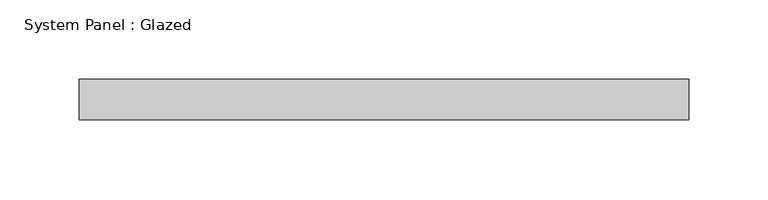
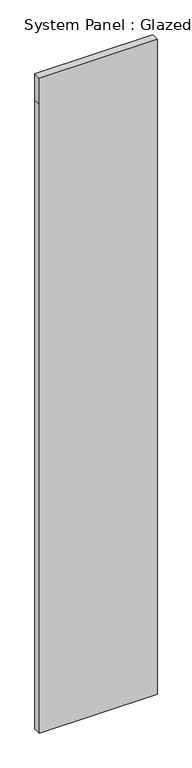
"""IFC4 building model written with IfcOpenShell, lengths in millimetres: plate geometry, System Panel : Glazed."""

import ifcopenshell
import ifcopenshell.guid

model = None  # the IFC model being written
_history = None  # IfcOwnerHistory: only IFC2X3 demands one
_inside = {}  # id of a spatial element -> (the spatial element, [elements in it])
_under = {}  # id of a project, library or spatial element -> (it, [spatial elements below it])
_declared = {}  # id of a project -> (the project, [libraries it declares])
_typed = {}  # id of a type object -> (the type object, [elements of that type])
_made_of = {}  # id of a material, layer set ... -> (it, [elements and type objects made of it])


def new_model(schema):
    """Start an empty IFC model of exactly this schema.

    Asked for "IFC4X3", IfcOpenShell would pick the latest addendum, in which some entities
    have other attributes; the version numbers below select the first issue.
    IFC2X3 requires an IfcOwnerHistory on every rooted entity: one is made here for all.
    """
    global model, _history
    if schema == "IFC4X3":
        model = ifcopenshell.file(schema_version=(4, 3, 0, 0))
    else:
        model = ifcopenshell.file(schema=schema)
    _inside.clear()
    _under.clear()
    _declared.clear()
    _typed.clear()
    _made_of.clear()
    _history = None
    if model.schema == "IFC2X3":
        org = make("IfcOrganization", Name="unknown")
        user = make(
            "IfcPersonAndOrganization",
            ThePerson=make("IfcPerson", FamilyName="unknown"),
            TheOrganization=org,
        )
        app = make(
            "IfcApplication",
            ApplicationDeveloper=org,
            Version="unknown",
            ApplicationFullName="unknown",
            ApplicationIdentifier="unknown",
        )
        _history = make(
            "IfcOwnerHistory",
            OwningUser=user,
            OwningApplication=app,
            ChangeAction="ADDED",
            CreationDate=0,
        )
    return model


def make(cls, **values):
    """One entity of the class cls with the attributes given. An attribute that is None is left unset."""
    return model.create_entity(
        cls, **{name: value for name, value in values.items() if value is not None}
    )


def rooted(cls, **values):
    """An entity with a GlobalId (a new one), such as an element, a storey or a relation."""
    return make(cls, GlobalId=ifcopenshell.guid.new(), OwnerHistory=_history, **values)


def si_unit(unit_type, name, prefix=None):
    """IfcSIUnit, for example si_unit("LENGTHUNIT", "METRE", prefix="MILLI")."""
    return make("IfcSIUnit", UnitType=unit_type, Prefix=prefix, Name=name)


def assignment(units):
    """IfcUnitAssignment: the units of a project."""
    return None if units is None else make("IfcUnitAssignment", Units=units)


def point(xyz):
    """IfcCartesianPoint."""
    return None if xyz is None else make("IfcCartesianPoint", Coordinates=xyz)


def direction(xyz):
    """IfcDirection."""
    return None if xyz is None else make("IfcDirection", DirectionRatios=xyz)


def frame(location, z_axis=None, x_axis=None):
    """IfcAxis2Placement3D, a coordinate frame: its origin and axes. An axis left out is left unset."""
    return make(
        "IfcAxis2Placement3D",
        Location=point(location),
        Axis=direction(z_axis),
        RefDirection=direction(x_axis),
    )


def origin():
    """The frame at (0, 0, 0) with its axes left unset."""
    return frame((0.0, 0.0, 0.0))


def place(relative_to, where):
    """IfcLocalPlacement: puts the frame where relative to a parent placement (None: the world)."""
    return make(
        "IfcLocalPlacement", PlacementRelTo=relative_to, RelativePlacement=where
    )


def context(
    kind, dimensions, precision=None, world=None, true_north=None, identifier=None
):
    """IfcGeometricRepresentationContext, for example the 3D "Model" context."""
    return make(
        "IfcGeometricRepresentationContext",
        ContextIdentifier=identifier,
        ContextType=kind,
        CoordinateSpaceDimension=dimensions,
        Precision=precision,
        WorldCoordinateSystem=world,
        TrueNorth=true_north,
    )


def project(units=None, contexts=None):
    """IfcProject with its units and contexts."""
    return rooted(
        "IfcProject",
        Name="project",
        RepresentationContexts=contexts,
        UnitsInContext=assignment(units),
    )


def spatial(cls, under=None, at=None, **own):
    """A site, building, storey or space (cls), placed at a placement, below another one or the project."""
    s = rooted(cls, ObjectPlacement=at, **own)
    if under is not None:
        _under.setdefault(under.id(), (under, []))[1].append(s)
    return s


def polyline(points):
    """IfcPolyline through the points."""
    return make("IfcPolyline", Points=[point(p) for p in points])


def outline(outer, holes=None, kind="AREA"):
    """IfcArbitraryClosedProfileDef: a profile drawn as a closed curve; with holes, ...WithVoids."""
    if holes is None:
        return make("IfcArbitraryClosedProfileDef", ProfileType=kind, OuterCurve=outer)
    return make(
        "IfcArbitraryProfileDefWithVoids",
        ProfileType=kind,
        OuterCurve=outer,
        InnerCurves=holes,
    )


def extrude(swept, where, along, depth):
    """IfcExtrudedAreaSolid: the profile swept, set in the frame where, extruded along a direction by depth."""
    return make(
        "IfcExtrudedAreaSolid",
        SweptArea=swept,
        Position=where,
        ExtrudedDirection=direction(along),
        Depth=depth,
    )


def shape(context_of_items, identifier, shape_type, items):
    """IfcShapeRepresentation: the items that make up one representation, for example the "Body"."""
    return make(
        "IfcShapeRepresentation",
        ContextOfItems=context_of_items,
        RepresentationIdentifier=identifier,
        RepresentationType=shape_type,
        Items=items,
    )


def source(mapping_origin, context_of_items, identifier, shape_type, items):
    """IfcRepresentationMap: a shape defined once, which mapped items show again and again."""
    return make(
        "IfcRepresentationMap",
        MappingOrigin=mapping_origin,
        MappedRepresentation=shape(context_of_items, identifier, shape_type, items),
    )


def transform(
    local_origin,
    x_axis=None,
    y_axis=None,
    z_axis=None,
    scale=None,
    scale2=None,
    scale3=None,
    uniform=True,
):
    """IfcCartesianTransformationOperator3D, or its non-uniform kind. x_axis, y_axis, z_axis: its Axis1, 2, 3."""
    if uniform:
        return make(
            "IfcCartesianTransformationOperator3D",
            Axis1=direction(x_axis),
            Axis2=direction(y_axis),
            LocalOrigin=point(local_origin),
            Scale=scale,
            Axis3=direction(z_axis),
        )
    return make(
        "IfcCartesianTransformationOperator3DnonUniform",
        Axis1=direction(x_axis),
        Axis2=direction(y_axis),
        LocalOrigin=point(local_origin),
        Scale=scale,
        Axis3=direction(z_axis),
        Scale2=scale2,
        Scale3=scale3,
    )


def mapped(mapping_source, mapping_target):
    """IfcMappedItem: shows the shape of a source again, moved by a transform."""
    return make(
        "IfcMappedItem", MappingSource=mapping_source, MappingTarget=mapping_target
    )


def made_of(thing, what):
    """Note that an element or type object is made of a material, layer set ...; save() writes the relation."""
    if what is not None:
        _made_of.setdefault(what.id(), (what, []))[1].append(thing)
    return thing


def element(
    cls,
    number,
    at=None,
    inside=None,
    cuts=None,
    type_object=None,
    material=None,
    context=None,
    identifier="Body",
    shape_type=None,
    held_by="IfcProductDefinitionShape",
    body=None,
    shapes=None,
    **own,
):
    """One element of the class cls, such as IfcWall. Its Tag is "e" and its number.

    at: its placement. inside: the storey or other place that contains it. cuts: it is an
    opening in that element (IfcRelVoidsElement). A single representation is given by context,
    identifier, shape_type and body (its items); several are given by shapes. held_by: the class
    of the entity that holds the representations. save() writes the other relations.
    """
    e = rooted(cls, Tag="e%d" % number, ObjectPlacement=at, **own)
    if body is not None:
        shapes = [shape(context, identifier, shape_type, body)]
    if shapes is not None:
        e.Representation = make(held_by, Representations=shapes)
    if inside is not None:
        _inside.setdefault(inside.id(), (inside, []))[1].append(e)
    if cuts is not None:
        rooted(
            "IfcRelVoidsElement", RelatingBuildingElement=cuts, RelatedOpeningElement=e
        )
    if type_object is not None:
        _typed.setdefault(type_object.id(), (type_object, []))[1].append(e)
    return made_of(e, material)


def aggregate(whole, parts):
    """IfcRelAggregates: a whole, such as a stair, and the parts it consists of."""
    return rooted("IfcRelAggregates", RelatingObject=whole, RelatedObjects=parts)


def save(model, path):
    """Write the relations noted so far, then the file.

    IfcRelAggregates (storeys below a building ...), IfcRelContainedInSpatialStructure (elements
    in a storey), IfcRelDefinesByType, IfcRelAssociatesMaterial and IfcRelDeclares: one each for
    every whole, place, type object, material and project.
    """
    for whole, parts in _under.values():
        aggregate(whole, parts)
    for where, things in _inside.values():
        rooted(
            "IfcRelContainedInSpatialStructure",
            RelatedElements=things,
            RelatingStructure=where,
        )
    for kind, things in _typed.values():
        rooted("IfcRelDefinesByType", RelatedObjects=things, RelatingType=kind)
    for what, things in _made_of.values():
        rooted("IfcRelAssociatesMaterial", RelatedObjects=things, RelatingMaterial=what)
    for by, libraries in _declared.values():
        rooted("IfcRelDeclares", RelatingContext=by, RelatedDefinitions=libraries)
    model.write(path)


def system_panel_glazed_6caf7cd9(model_context):
    return source(origin(), model_context, "Body", "SweptSolid", [
        extrude(outline(polyline([(0.0, -192.1303048), (0.0, 192.1303048), (2171.7, 192.1303048), (2260.6, 192.1303048), (2260.6, -192.1303048), (2171.7, -192.1303048), (0.0, -192.1303048)])), frame((0.0, 19.05, 0.0), z_axis=(0.0, 1.0, 0.0), x_axis=(0.0, 0.0, 1.0)), (0.0, 0.0, 1.0), 25.4),
    ])


if __name__ == "__main__":
    model = new_model("IFC4")
    model_context = context("Model", 3, world=origin())
    ifc_project = project(units=[si_unit("LENGTHUNIT", "METRE", prefix="MILLI")], contexts=[model_context])
    site = spatial("IfcSite", under=ifc_project)
    building = spatial("IfcBuilding", under=site)
    placement = place(None, origin())
    system_panel_glazed_shape = system_panel_glazed_6caf7cd9(model_context)
    element("IfcPlate", 1, ObjectType="System Panel : Glazed", at=placement, inside=building, context=model_context, shape_type="MappedRepresentation", body=[
        mapped(system_panel_glazed_shape, transform((0.0, 0.0, 0.0), x_axis=(1.0, 0.0, 0.0), y_axis=(0.0, 1.0, 0.0), z_axis=(0.0, 0.0, 1.0))),
    ])
    save(model, "model.ifc")

# Revit data of these elements
# Element 1 (IfcPlate, "System Panel : Glazed")
#   Materials on its faces: "Glass"
# Materials
#   "Glass": class "Glass", colour RGB 218 227 224, transparency 0.85, Description = "Soda Lime Glass", Cost = 0
